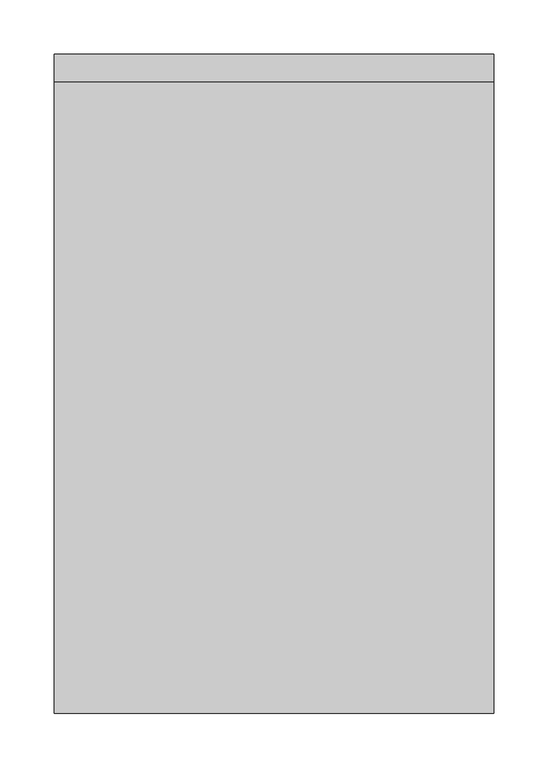
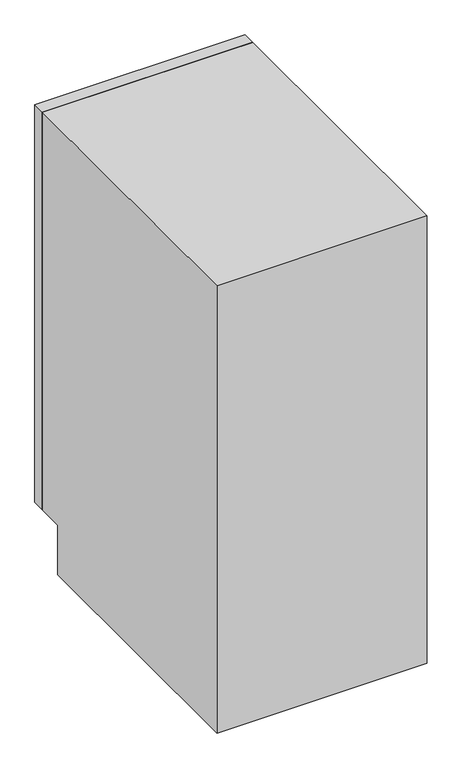
"""IFC4 building model written with IfcOpenShell, lengths in millimetres: furniture geometry, OD_CW_Base Cabinet : OD_CW_Base Cabinet."""

from ifc_helpers import new_model, si_unit, frame, origin, place, context, project, spatial, polyline, outline, extrude, source, transform, mapped, element, save


def furniture_ab8d68fc(model_context):
    return source(origin(), model_context, "Body", "SweptSolid", [
        extrude(outline(polyline([(18.7377049, -25.4), (18.7377049, 0.0), (425.1377049, 0.0), (425.1377049, -25.4), (18.7377049, -25.4)])), frame((0.0, 0.0, 101.6), z_axis=(0.0, 0.0, 1.0), x_axis=(1.0, 0.0, 0.0)), (0.0, 0.0, 1.0), 812.8),
        extrude(outline(polyline([(-25.4, 914.4), (-25.4, 101.6), (-76.2, 101.6), (-76.2, 0.0), (-609.6, 0.0), (-609.6, 914.4), (-25.4, 914.4)])), frame((18.7377049, 0.0, 0.0), z_axis=(1.0, 0.0, 0.0), x_axis=(0.0, 1.0, 0.0)), (0.0, 0.0, 1.0), 406.4),
    ])


if __name__ == "__main__":
    model = new_model("IFC4")
    model_context = context("Model", 3, world=origin())
    ifc_project = project(units=[si_unit("LENGTHUNIT", "METRE", prefix="MILLI")], contexts=[model_context])
    site = spatial("IfcSite", under=ifc_project)
    building = spatial("IfcBuilding", under=site)
    placement = place(None, origin())
    furniture_shape = furniture_ab8d68fc(model_context)
    element("IfcFurniture", 1, ObjectType="OD_CW_Base Cabinet : OD_CW_Base Cabinet", at=placement, inside=building, context=model_context, shape_type="MappedRepresentation", body=[
        mapped(furniture_shape, transform((0.0, 0.0, 0.0), x_axis=(1.0, 0.0, 0.0), y_axis=(0.0, 1.0, 0.0), z_axis=(0.0, 0.0, 1.0))),
    ])
    save(model, "model.ifc")

# Revit data of these elements
# Type "OD_CW_Base Cabinet : OD_CW_Base Cabinet"
#   OD_CW_Width [instance default] = 2' - 10"
#   OD_CW_Length [instance default] = 8' - 0"
#   OD_CW_Height [instance default] = 2' - 3"
#   Depth = 2' - 0"
#   Height = 3' - 0"
#   Width = 4' - 0"
#   OD_CW_Material_Front Panel [instance default] = none
#   OD_CW_Material_Body [instance default] = none
# Element 1 (IfcFurniture, "OD_CW_Base Cabinet : OD_CW_Base Cabinet")
#   OD_CW_Width = 2' - 0"
#   OD_CW_Length = 1' - 4"
#   OD_CW_Height = 3' - 0"
#   OD_CW_Material_Body = DOUGH TRAY
#   Materials on its faces: "DOUGH TRAY", "CASEWORK"
# Materials
#   "DOUGH TRAY": class "Generic", colour RGB 187 187 187, transparency 0, Cost = 0
#   "CASEWORK": class "Generic", colour RGB 181 181 181, transparency 0, Cost = 0
